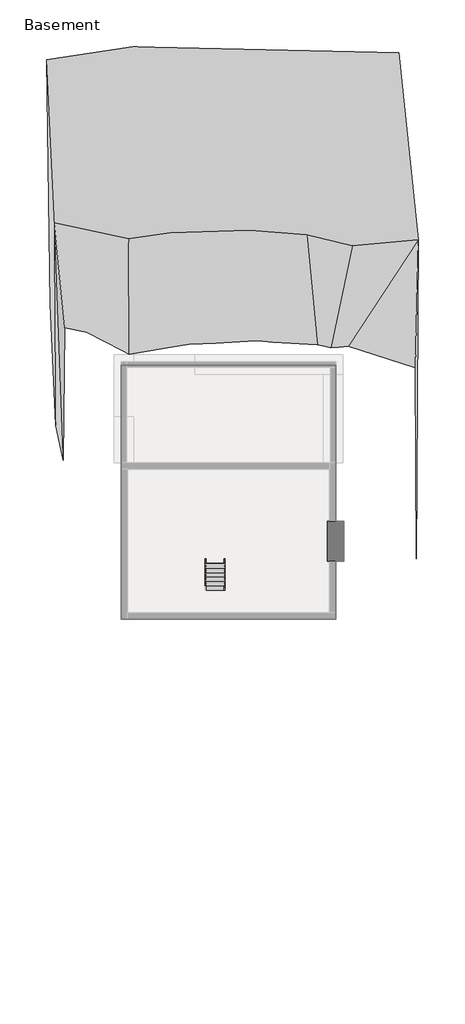
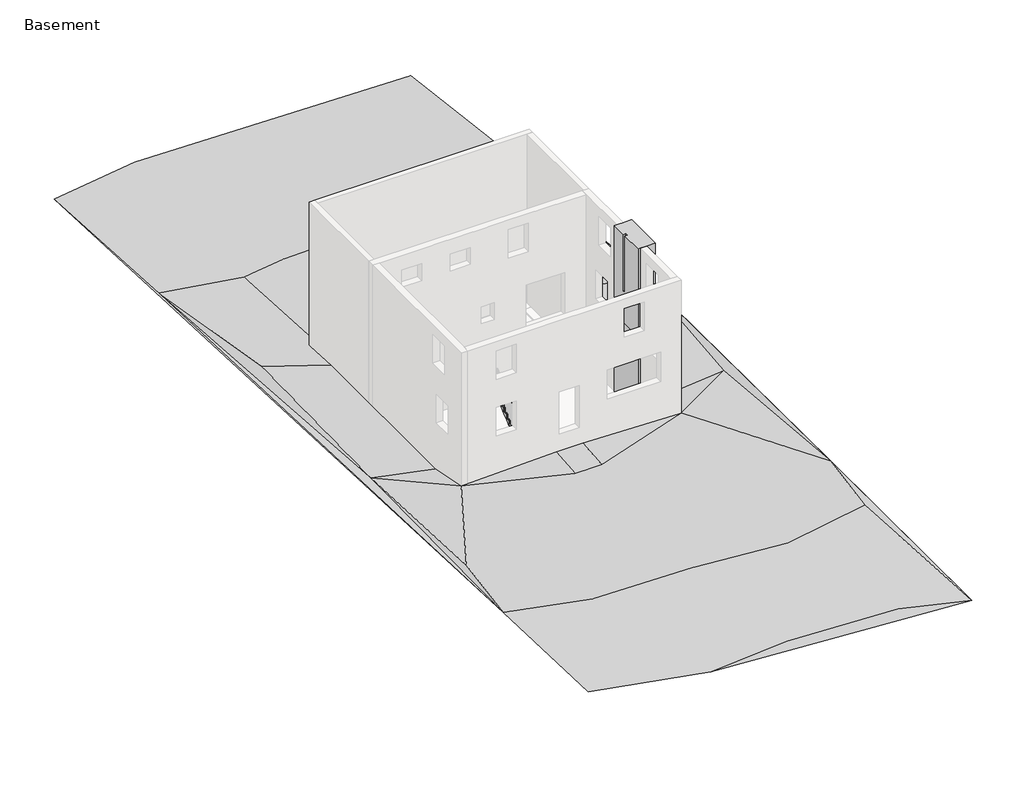
# One storey, part 2 of 2: 4 proxies, 2 members, 1 railing, 1 stair flight.
"""IFC4 building model written with IfcOpenShell, lengths in millimetres."""

import ifcopenshell
import ifcopenshell.guid

model = None  # the IFC model being written
_history = None  # IfcOwnerHistory: only IFC2X3 demands one
_inside = {}  # id of a spatial element -> (the spatial element, [elements in it])
_under = {}  # id of a project, library or spatial element -> (it, [spatial elements below it])
_declared = {}  # id of a project -> (the project, [libraries it declares])
_typed = {}  # id of a type object -> (the type object, [elements of that type])
_made_of = {}  # id of a material, layer set ... -> (it, [elements and type objects made of it])


def new_model(schema):
    """Start an empty IFC model of exactly this schema.

    Asked for "IFC4X3", IfcOpenShell would pick the latest addendum, in which some entities
    have other attributes; the version numbers below select the first issue.
    IFC2X3 requires an IfcOwnerHistory on every rooted entity: one is made here for all.
    """
    global model, _history
    if schema == "IFC4X3":
        model = ifcopenshell.file(schema_version=(4, 3, 0, 0))
    else:
        model = ifcopenshell.file(schema=schema)
    _inside.clear()
    _under.clear()
    _declared.clear()
    _typed.clear()
    _made_of.clear()
    _history = None
    if model.schema == "IFC2X3":
        org = make("IfcOrganization", Name="unknown")
        user = make(
            "IfcPersonAndOrganization",
            ThePerson=make("IfcPerson", FamilyName="unknown"),
            TheOrganization=org,
        )
        app = make(
            "IfcApplication",
            ApplicationDeveloper=org,
            Version="unknown",
            ApplicationFullName="unknown",
            ApplicationIdentifier="unknown",
        )
        _history = make(
            "IfcOwnerHistory",
            OwningUser=user,
            OwningApplication=app,
            ChangeAction="ADDED",
            CreationDate=0,
        )
    return model


def make(cls, **values):
    """One entity of the class cls with the attributes given. An attribute that is None is left unset."""
    return model.create_entity(
        cls, **{name: value for name, value in values.items() if value is not None}
    )


def rooted(cls, **values):
    """An entity with a GlobalId (a new one), such as an element, a storey or a relation."""
    return make(cls, GlobalId=ifcopenshell.guid.new(), OwnerHistory=_history, **values)


def si_unit(unit_type, name, prefix=None):
    """IfcSIUnit, for example si_unit("LENGTHUNIT", "METRE", prefix="MILLI")."""
    return make("IfcSIUnit", UnitType=unit_type, Prefix=prefix, Name=name)


def assignment(units):
    """IfcUnitAssignment: the units of a project."""
    return None if units is None else make("IfcUnitAssignment", Units=units)


def point(xyz):
    """IfcCartesianPoint."""
    return None if xyz is None else make("IfcCartesianPoint", Coordinates=xyz)


def direction(xyz):
    """IfcDirection."""
    return None if xyz is None else make("IfcDirection", DirectionRatios=xyz)


def frame(location, z_axis=None, x_axis=None):
    """IfcAxis2Placement3D, a coordinate frame: its origin and axes. An axis left out is left unset."""
    return make(
        "IfcAxis2Placement3D",
        Location=point(location),
        Axis=direction(z_axis),
        RefDirection=direction(x_axis),
    )


def origin():
    """The frame at (0, 0, 0) with its axes left unset."""
    return frame((0.0, 0.0, 0.0))


def place(relative_to, where):
    """IfcLocalPlacement: puts the frame where relative to a parent placement (None: the world)."""
    return make(
        "IfcLocalPlacement", PlacementRelTo=relative_to, RelativePlacement=where
    )


def context(
    kind, dimensions, precision=None, world=None, true_north=None, identifier=None
):
    """IfcGeometricRepresentationContext, for example the 3D "Model" context."""
    return make(
        "IfcGeometricRepresentationContext",
        ContextIdentifier=identifier,
        ContextType=kind,
        CoordinateSpaceDimension=dimensions,
        Precision=precision,
        WorldCoordinateSystem=world,
        TrueNorth=true_north,
    )


def project(units=None, contexts=None):
    """IfcProject with its units and contexts."""
    return rooted(
        "IfcProject",
        Name="project",
        RepresentationContexts=contexts,
        UnitsInContext=assignment(units),
    )


def spatial(cls, under=None, at=None, **own):
    """A site, building, storey or space (cls), placed at a placement, below another one or the project."""
    s = rooted(cls, ObjectPlacement=at, **own)
    if under is not None:
        _under.setdefault(under.id(), (under, []))[1].append(s)
    return s


def polyline(points):
    """IfcPolyline through the points."""
    return make("IfcPolyline", Points=[point(p) for p in points])


def point_list(points):
    """IfcCartesianPointList2D or 3D."""
    cls = (
        "IfcCartesianPointList2D" if len(points[0]) == 2 else "IfcCartesianPointList3D"
    )
    return make(cls, CoordList=points)


def outline(outer, holes=None, kind="AREA"):
    """IfcArbitraryClosedProfileDef: a profile drawn as a closed curve; with holes, ...WithVoids."""
    if holes is None:
        return make("IfcArbitraryClosedProfileDef", ProfileType=kind, OuterCurve=outer)
    return make(
        "IfcArbitraryProfileDefWithVoids",
        ProfileType=kind,
        OuterCurve=outer,
        InnerCurves=holes,
    )


def extrude(swept, where, along, depth):
    """IfcExtrudedAreaSolid: the profile swept, set in the frame where, extruded along a direction by depth."""
    return make(
        "IfcExtrudedAreaSolid",
        SweptArea=swept,
        Position=where,
        ExtrudedDirection=direction(along),
        Depth=depth,
    )


def faces_of(points, faces, orient=None, outer=None):
    """IfcFace entities. A face is a list of loops; a loop is a list of indices into points, from 0.

    orient and outer hold one flag for each loop. By default every Orientation is true, the
    first loop of a face is its IfcFaceOuterBound and the others are IfcFaceBound.
    """
    made = []
    for i, loops in enumerate(faces):
        bounds = []
        for j, loop in enumerate(loops):
            is_outer = j == 0 if outer is None else outer[i][j]
            bounds.append(
                make(
                    "IfcFaceOuterBound" if is_outer else "IfcFaceBound",
                    Bound=make("IfcPolyLoop", Polygon=[points[k] for k in loop]),
                    Orientation=True if orient is None else orient[i][j],
                )
            )
        made.append(make("IfcFace", Bounds=bounds))
    return made


def faceted_brep(points, faces, orient=None, outer=None, voids=None):
    """IfcFacetedBrep: a solid bounded by flat faces; with voids (closed shells), ...WithVoids."""
    shared = [point(p) for p in points]
    hull = make("IfcClosedShell", CfsFaces=faces_of(shared, faces, orient, outer))
    if voids is None:
        return make("IfcFacetedBrep", Outer=hull)
    return make(
        "IfcFacetedBrepWithVoids",
        Outer=hull,
        Voids=[
            make(cls, CfsFaces=faces_of(shared, fs, o, b)) for cls, fs, o, b in voids
        ],
    )


def triangles(points, corners, closed=None, point_numbers=None):
    """IfcTriangulatedFaceSet: each triangle names its three corners, points numbered from 1."""
    return make(
        "IfcTriangulatedFaceSet",
        Coordinates=point_list(points),
        Closed=closed,
        CoordIndex=corners,
        PnIndex=point_numbers,
    )


def shape(context_of_items, identifier, shape_type, items):
    """IfcShapeRepresentation: the items that make up one representation, for example the "Body"."""
    return make(
        "IfcShapeRepresentation",
        ContextOfItems=context_of_items,
        RepresentationIdentifier=identifier,
        RepresentationType=shape_type,
        Items=items,
    )


def source(mapping_origin, context_of_items, identifier, shape_type, items):
    """IfcRepresentationMap: a shape defined once, which mapped items show again and again."""
    return make(
        "IfcRepresentationMap",
        MappingOrigin=mapping_origin,
        MappedRepresentation=shape(context_of_items, identifier, shape_type, items),
    )


def transform(
    local_origin,
    x_axis=None,
    y_axis=None,
    z_axis=None,
    scale=None,
    scale2=None,
    scale3=None,
    uniform=True,
):
    """IfcCartesianTransformationOperator3D, or its non-uniform kind. x_axis, y_axis, z_axis: its Axis1, 2, 3."""
    if uniform:
        return make(
            "IfcCartesianTransformationOperator3D",
            Axis1=direction(x_axis),
            Axis2=direction(y_axis),
            LocalOrigin=point(local_origin),
            Scale=scale,
            Axis3=direction(z_axis),
        )
    return make(
        "IfcCartesianTransformationOperator3DnonUniform",
        Axis1=direction(x_axis),
        Axis2=direction(y_axis),
        LocalOrigin=point(local_origin),
        Scale=scale,
        Axis3=direction(z_axis),
        Scale2=scale2,
        Scale3=scale3,
    )


def mapped(mapping_source, mapping_target):
    """IfcMappedItem: shows the shape of a source again, moved by a transform."""
    return make(
        "IfcMappedItem", MappingSource=mapping_source, MappingTarget=mapping_target
    )


def made_of(thing, what):
    """Note that an element or type object is made of a material, layer set ...; save() writes the relation."""
    if what is not None:
        _made_of.setdefault(what.id(), (what, []))[1].append(thing)
    return thing


def element(
    cls,
    number,
    at=None,
    inside=None,
    cuts=None,
    type_object=None,
    material=None,
    context=None,
    identifier="Body",
    shape_type=None,
    held_by="IfcProductDefinitionShape",
    body=None,
    shapes=None,
    **own,
):
    """One element of the class cls, such as IfcWall. Its Tag is "e" and its number.

    at: its placement. inside: the storey or other place that contains it. cuts: it is an
    opening in that element (IfcRelVoidsElement). A single representation is given by context,
    identifier, shape_type and body (its items); several are given by shapes. held_by: the class
    of the entity that holds the representations. save() writes the other relations.
    """
    e = rooted(cls, Tag="e%d" % number, ObjectPlacement=at, **own)
    if body is not None:
        shapes = [shape(context, identifier, shape_type, body)]
    if shapes is not None:
        e.Representation = make(held_by, Representations=shapes)
    if inside is not None:
        _inside.setdefault(inside.id(), (inside, []))[1].append(e)
    if cuts is not None:
        rooted(
            "IfcRelVoidsElement", RelatingBuildingElement=cuts, RelatedOpeningElement=e
        )
    if type_object is not None:
        _typed.setdefault(type_object.id(), (type_object, []))[1].append(e)
    return made_of(e, material)


def aggregate(whole, parts):
    """IfcRelAggregates: a whole, such as a stair, and the parts it consists of."""
    return rooted("IfcRelAggregates", RelatingObject=whole, RelatedObjects=parts)


def save(model, path):
    """Write the relations noted so far, then the file.

    IfcRelAggregates (storeys below a building ...), IfcRelContainedInSpatialStructure (elements
    in a storey), IfcRelDefinesByType, IfcRelAssociatesMaterial and IfcRelDeclares: one each for
    every whole, place, type object, material and project.
    """
    for whole, parts in _under.values():
        aggregate(whole, parts)
    for where, things in _inside.values():
        rooted(
            "IfcRelContainedInSpatialStructure",
            RelatedElements=things,
            RelatingStructure=where,
        )
    for kind, things in _typed.values():
        rooted("IfcRelDefinesByType", RelatedObjects=things, RelatingType=kind)
    for what, things in _made_of.values():
        rooted("IfcRelAssociatesMaterial", RelatedObjects=things, RelatingMaterial=what)
    for by, libraries in _declared.values():
        rooted("IfcRelDeclares", RelatingContext=by, RelatedDefinitions=libraries)
    model.write(path)


def existing_fireplace_existing_fireplace_063a625f(model_context):
    return source(origin(), model_context, "Body", "Brep", [
        faceted_brep([(4450.2196932, 434.2888758, 5486.4), (4069.2196932, 434.2888758, 5486.4), (3764.4196932, 434.2888758, 5486.4), (3662.8196932, 434.2888758, 5486.4), (3662.8196932, -276.9111242, 5486.4), (3767.2567114, -276.9111242, 5486.4), (3767.2567114, -403.9111242, 5486.4), (3662.8196932, -403.9111242, 5486.4), (3662.8196932, -1445.3111242, 5486.4), (3764.4196932, -1445.3111242, 5486.4), (4069.2196932, -1445.3111242, 5486.4), (4450.2196932, -1445.3111242, 5486.4), (4450.2196932, 434.2888758, -2667.0), (4450.2196932, -1445.3111242, -2667.0), (4069.2196932, -1445.3111242, -2667.0), (3764.4196932, -1445.3111242, -2667.0), (3662.8196932, -1445.3111242, -2667.0), (3662.8196932, 434.2888758, -2667.0), (3764.4196932, 434.2888758, -2667.0), (4069.2196932, 434.2888758, -2667.0), (3662.8196932, -403.9111242, 2743.2), (3662.8196932, -276.9111242, 2743.2), (3662.8196932, 154.8888758, 0.0), (3662.8196932, 154.8888758, 1219.2), (3662.8196932, -1165.9111242, 1219.2), (3662.8196932, -1165.9111242, 0.0), (4145.4196932, -20.7631592, 1219.2), (4145.4196932, -990.2590891, 1219.2), (4145.4196932, -990.2590891, 0.0), (4145.4196932, -20.7631592, 0.0), (3767.2567114, -403.9111242, 2743.2), (3767.2567114, -276.9111242, 2743.2)], [[[0, 1, 2, 3, 4, 5, 6, 7, 8, 9, 10, 11]], [[12, 13, 14, 15, 16, 17, 18, 19]], [[3, 2, 1, 0, 12, 19, 18, 17]], [[3, 17, 16, 8, 7, 20, 21, 4], [22, 23, 24, 25]], [[11, 10, 9, 8, 16, 15, 14, 13]], [[0, 11, 13, 12]], [[24, 23, 26, 27]], [[25, 24, 27, 28]], [[27, 26, 29, 28]], [[23, 22, 29, 26]], [[22, 25, 28, 29]], [[6, 30, 20, 7]], [[31, 5, 4, 21]], [[30, 31, 21, 20]], [[30, 6, 5, 31]]]),
    ])


def stair_flight_b746b64e(model_context):
    return source(origin(), model_context, "Body", "SweptSolid", [
        extrude(outline(polyline([(-2791.5111242, -2476.5), (-2562.9111242, -2476.5), (-2562.9111242, -2527.3), (-2766.1111242, -2527.3), (-2766.1111242, -2520.95), (-2791.5111242, -2495.55), (-2791.5111242, -2476.5)])), frame((-2052.1803068, 0.0, 0.0), z_axis=(1.0, 0.0, 0.0), x_axis=(0.0, 1.0, 0.0)), (0.0, 0.0, 1.0), 939.8),
        extrude(outline(polyline([(-1112.3803068, -2759.7611242), (-1112.3803068, -2766.1111242), (-2052.1803068, -2766.1111242), (-2052.1803068, -2759.7611242), (-1112.3803068, -2759.7611242)])), frame((0.0, 0.0, -2667.0), z_axis=(0.0, 0.0, 1.0), x_axis=(1.0, 0.0, 0.0)), (0.0, 0.0, 1.0), 139.7),
        extrude(outline(polyline([(-1112.3803068, -2556.5611242), (-1112.3803068, -2562.9111242), (-2052.1803068, -2562.9111242), (-2052.1803068, -2556.5611242), (-1112.3803068, -2556.5611242)])), frame((0.0, 0.0, -2527.3), z_axis=(0.0, 0.0, 1.0), x_axis=(1.0, 0.0, 0.0)), (0.0, 0.0, 1.0), 190.5),
        extrude(outline(polyline([(-2588.3111242, -2286.0), (-2359.7111242, -2286.0), (-2359.7111242, -2336.8), (-2562.9111242, -2336.8), (-2562.9111242, -2330.45), (-2588.3111242, -2305.05), (-2588.3111242, -2286.0)])), frame((-2052.1803068, 0.0, 0.0), z_axis=(1.0, 0.0, 0.0), x_axis=(0.0, 1.0, 0.0)), (0.0, 0.0, 1.0), 939.8),
        extrude(outline(polyline([(-1112.3803068, -2353.3611242), (-1112.3803068, -2359.7111242), (-2052.1803068, -2359.7111242), (-2052.1803068, -2353.3611242), (-1112.3803068, -2353.3611242)])), frame((0.0, 0.0, -2336.8), z_axis=(0.0, 0.0, 1.0), x_axis=(1.0, 0.0, 0.0)), (0.0, 0.0, 1.0), 190.5),
        extrude(outline(polyline([(-2385.1111242, -2095.5), (-2156.5111242, -2095.5), (-2156.5111242, -2146.3), (-2359.7111242, -2146.3), (-2359.7111242, -2139.95), (-2385.1111242, -2114.55), (-2385.1111242, -2095.5)])), frame((-2052.1803068, 0.0, 0.0), z_axis=(1.0, 0.0, 0.0), x_axis=(0.0, 1.0, 0.0)), (0.0, 0.0, 1.0), 939.8),
        extrude(outline(polyline([(-1112.3803068, -2150.1611242), (-1112.3803068, -2156.5111242), (-2052.1803068, -2156.5111242), (-2052.1803068, -2150.1611242), (-1112.3803068, -2150.1611242)])), frame((0.0, 0.0, -2146.3), z_axis=(0.0, 0.0, 1.0), x_axis=(1.0, 0.0, 0.0)), (0.0, 0.0, 1.0), 190.5),
        extrude(outline(polyline([(-2181.9111242, -1905.0), (-1953.3111242, -1905.0), (-1953.3111242, -1955.8), (-2156.5111242, -1955.8), (-2156.5111242, -1949.45), (-2181.9111242, -1924.05), (-2181.9111242, -1905.0)])), frame((-2052.1803068, 0.0, 0.0), z_axis=(1.0, 0.0, 0.0), x_axis=(0.0, 1.0, 0.0)), (0.0, 0.0, 1.0), 939.8),
        extrude(outline(polyline([(-1112.3803068, -1946.9611242), (-1112.3803068, -1953.3111242), (-2052.1803068, -1953.3111242), (-2052.1803068, -1946.9611242), (-1112.3803068, -1946.9611242)])), frame((0.0, 0.0, -1955.8), z_axis=(0.0, 0.0, 1.0), x_axis=(1.0, 0.0, 0.0)), (0.0, 0.0, 1.0), 190.5),
        extrude(outline(polyline([(-1978.7111242, -1714.5), (-1750.1111242, -1714.5), (-1750.1111242, -1765.3), (-1953.3111242, -1765.3), (-1953.3111242, -1758.95), (-1978.7111242, -1733.55), (-1978.7111242, -1714.5)])), frame((-2052.1803068, 0.0, 0.0), z_axis=(1.0, 0.0, 0.0), x_axis=(0.0, 1.0, 0.0)), (0.0, 0.0, 1.0), 939.8),
        extrude(outline(polyline([(-1112.3803068, -1743.7611242), (-1112.3803068, -1750.1111242), (-2052.1803068, -1750.1111242), (-2052.1803068, -1743.7611242), (-1112.3803068, -1743.7611242)])), frame((0.0, 0.0, -1765.3), z_axis=(0.0, 0.0, 1.0), x_axis=(1.0, 0.0, 0.0)), (0.0, 0.0, 1.0), 190.5),
        extrude(outline(polyline([(-1775.5111242, -1524.0), (-1546.9111242, -1524.0), (-1546.9111242, -1574.8), (-1750.1111242, -1574.8), (-1750.1111242, -1568.45), (-1775.5111242, -1543.05), (-1775.5111242, -1524.0)])), frame((-2052.1803068, 0.0, 0.0), z_axis=(1.0, 0.0, 0.0), x_axis=(0.0, 1.0, 0.0)), (0.0, 0.0, 1.0), 939.8),
        extrude(outline(polyline([(-1112.3803068, -1540.5611242), (-1112.3803068, -1546.9111242), (-2052.1803068, -1546.9111242), (-2052.1803068, -1540.5611242), (-1112.3803068, -1540.5611242)])), frame((0.0, 0.0, -1574.8), z_axis=(0.0, 0.0, 1.0), x_axis=(1.0, 0.0, 0.0)), (0.0, 0.0, 1.0), 190.5),
        extrude(outline(polyline([(-1572.3111242, -1333.5), (-1343.7111242, -1333.5), (-1343.7111242, -1384.3), (-1546.9111242, -1384.3), (-1546.9111242, -1377.95), (-1572.3111242, -1352.55), (-1572.3111242, -1333.5)])), frame((-2052.1803068, 0.0, 0.0), z_axis=(1.0, 0.0, 0.0), x_axis=(0.0, 1.0, 0.0)), (0.0, 0.0, 1.0), 939.8),
        extrude(outline(polyline([(-1112.3803068, -1337.3611242), (-1112.3803068, -1343.7111242), (-2052.1803068, -1343.7111242), (-2052.1803068, -1337.3611242), (-1112.3803068, -1337.3611242)])), frame((0.0, 0.0, -1384.3), z_axis=(0.0, 0.0, 1.0), x_axis=(1.0, 0.0, 0.0)), (0.0, 0.0, 1.0), 190.5),
        extrude(outline(polyline([(-1369.1111242, -1143.0), (-1140.5111242, -1143.0), (-1140.5111242, -1193.8), (-1343.7111242, -1193.8), (-1343.7111242, -1187.45), (-1369.1111242, -1162.05), (-1369.1111242, -1143.0)])), frame((-2052.1803068, 0.0, 0.0), z_axis=(1.0, 0.0, 0.0), x_axis=(0.0, 1.0, 0.0)), (0.0, 0.0, 1.0), 939.8),
        extrude(outline(polyline([(-1112.3803068, -1134.1611242), (-1112.3803068, -1140.5111242), (-2052.1803068, -1140.5111242), (-2052.1803068, -1134.1611242), (-1112.3803068, -1134.1611242)])), frame((0.0, 0.0, -1193.8), z_axis=(0.0, 0.0, 1.0), x_axis=(1.0, 0.0, 0.0)), (0.0, 0.0, 1.0), 190.5),
        extrude(outline(polyline([(-1165.9111242, -952.5), (-937.3111242, -952.5), (-937.3111242, -1003.3), (-1140.5111242, -1003.3), (-1140.5111242, -996.95), (-1165.9111242, -971.55), (-1165.9111242, -952.5)])), frame((-2052.1803068, 0.0, 0.0), z_axis=(1.0, 0.0, 0.0), x_axis=(0.0, 1.0, 0.0)), (0.0, 0.0, 1.0), 939.8),
        extrude(outline(polyline([(-1112.3803068, -930.9611242), (-1112.3803068, -937.3111242), (-2052.1803068, -937.3111242), (-2052.1803068, -930.9611242), (-1112.3803068, -930.9611242)])), frame((0.0, 0.0, -1003.3), z_axis=(0.0, 0.0, 1.0), x_axis=(1.0, 0.0, 0.0)), (0.0, 0.0, 1.0), 190.5),
        extrude(outline(polyline([(-962.7111242, -762.0), (-734.1111242, -762.0), (-734.1111242, -812.8), (-937.3111242, -812.8), (-937.3111242, -806.45), (-962.7111242, -781.05), (-962.7111242, -762.0)])), frame((-2052.1803068, 0.0, 0.0), z_axis=(1.0, 0.0, 0.0), x_axis=(0.0, 1.0, 0.0)), (0.0, 0.0, 1.0), 939.8),
        extrude(outline(polyline([(-1112.3803068, -727.7611242), (-1112.3803068, -734.1111242), (-2052.1803068, -734.1111242), (-2052.1803068, -727.7611242), (-1112.3803068, -727.7611242)])), frame((0.0, 0.0, -812.8), z_axis=(0.0, 0.0, 1.0), x_axis=(1.0, 0.0, 0.0)), (0.0, 0.0, 1.0), 190.5),
        extrude(outline(polyline([(-759.5111242, -571.5), (-530.9111242, -571.5), (-530.9111242, -622.3), (-734.1111242, -622.3), (-734.1111242, -615.95), (-759.5111242, -590.55), (-759.5111242, -571.5)])), frame((-2052.1803068, 0.0, 0.0), z_axis=(1.0, 0.0, 0.0), x_axis=(0.0, 1.0, 0.0)), (0.0, 0.0, 1.0), 939.8),
        extrude(outline(polyline([(-1112.3803068, -524.5611242), (-1112.3803068, -530.9111242), (-2052.1803068, -530.9111242), (-2052.1803068, -524.5611242), (-1112.3803068, -524.5611242)])), frame((0.0, 0.0, -622.3), z_axis=(0.0, 0.0, 1.0), x_axis=(1.0, 0.0, 0.0)), (0.0, 0.0, 1.0), 190.5),
        extrude(outline(polyline([(-556.3111242, -381.0), (-327.7111242, -381.0), (-327.7111242, -431.8), (-530.9111242, -431.8), (-530.9111242, -425.45), (-556.3111242, -400.05), (-556.3111242, -381.0)])), frame((-2052.1803068, 0.0, 0.0), z_axis=(1.0, 0.0, 0.0), x_axis=(0.0, 1.0, 0.0)), (0.0, 0.0, 1.0), 939.8),
        extrude(outline(polyline([(-1112.3803068, -321.3611242), (-1112.3803068, -327.7111242), (-2052.1803068, -327.7111242), (-2052.1803068, -321.3611242), (-1112.3803068, -321.3611242)])), frame((0.0, 0.0, -431.8), z_axis=(0.0, 0.0, 1.0), x_axis=(1.0, 0.0, 0.0)), (0.0, 0.0, 1.0), 190.5),
        extrude(outline(polyline([(-353.1111242, -190.5), (-124.5111242, -190.5), (-124.5111242, -241.3), (-327.7111242, -241.3), (-327.7111242, -234.95), (-353.1111242, -209.55), (-353.1111242, -190.5)])), frame((-2052.1803068, 0.0, 0.0), z_axis=(1.0, 0.0, 0.0), x_axis=(0.0, 1.0, 0.0)), (0.0, 0.0, 1.0), 939.8),
        extrude(outline(polyline([(-1112.3803068, -118.1611242), (-1112.3803068, -124.5111242), (-2052.1803068, -124.5111242), (-2052.1803068, -118.1611242), (-1112.3803068, -118.1611242)])), frame((0.0, 0.0, -241.3), z_axis=(0.0, 0.0, 1.0), x_axis=(1.0, 0.0, 0.0)), (0.0, 0.0, 1.0), 190.5),
    ])


model = new_model("IFC4")

# Units and contexts
model_context = context("Model", 3, world=origin())
ifc_project = project(units=[si_unit("LENGTHUNIT", "METRE", prefix="MILLI")], contexts=[model_context])

# Site, building, storey
site = spatial("IfcSite", under=ifc_project)
building = spatial("IfcBuilding", under=site)
storey = spatial("IfcBuildingStorey", under=building, Name="Basement", Elevation=-2667.0)

# Proxies
placement = place(None, origin())
element("IfcBuildingElementProxy", 1, Name="Building Element Proxy", at=placement, inside=storey, context=model_context, shape_type="Tessellation", body=[
    triangles([(-9474.14729, 22003.2871765, -1727.1999516), (-8916.1412338, -12566.1132111, -939.7999758), (-8632.7724838, -18803.3999359, -1092.1999758), (-3754.3850807, -20036.8885986, -1092.1999758), (7677.2023224, -20906.8378235, -1092.1999758), (7936.7585724, 13587.9496765, -1752.6), (7012.0400162, 22339.8364014, -1727.1999516), (-5437.1349838, 22620.8239014, -1727.1999516), (4069.2196426, 434.2888621, -1346.1999516), (4450.2196426, 434.2888621, -1346.1999516), (4450.2196426, -349.5066825, -1346.1999516), (4450.2196426, -1445.3110531, -1346.1999516), (4069.2196426, -1445.3110531, -1346.1999516), (4069.2196426, -2313.9084709, -1346.1999516), (4069.2196426, -4163.1110046, -939.7999758), (-426.580321, -4163.1110046, -812.8000242), (-1645.7803574, -4163.1110046, -812.8000242), (-5989.1803574, -4163.1110046, -939.7999758), (-5989.1803574, -2124.4043404, -1346.1999516), (-5989.1803574, 3152.0889954, -1346.1999516), (-5989.1803574, 4989.0600082, -1346.1999516), (-5989.1803574, 6156.3282944, -1346.1999516), (-5989.1803574, 7724.0889954, -1429.2445919), (-5611.7969971, 7724.0889954, -1439.6358181), (-2815.8938187, 7724.0889954, -1415.0254017), (-2474.4123367, 7724.0889954, -1412.4145145), (-1876.9665367, 7724.0889954, -1411.4359406), (391.3462071, 7724.0889954, -1403.6252254), (781.867392, 7724.0889954, -1405.4288944), (3306.7437996, 7724.0889954, -1413.4377079), (3676.8014442, 7724.0889954, -1418.4369667), (4069.2196426, 7724.0889954, -1416.2554138), (4069.2196426, 7529.9159637, -1404.4058464), (4069.2196426, 6299.0253983, -1346.1999516), (4069.2196426, 3152.0889954, -1346.1999516), (-9109.81604, 14372.1750641, -1752.6), (-8549.4287338, -9013.2876297, -939.7999758), (-8523.2349838, -1401.2252266, -1346.1999516), (-8408.9349838, 7414.1625641, -1346.1999516), (-6082.4537338, -10022.9382111, -939.7999758), (-5633.19104, 13643.5125641, -1752.6), (-5382.3662338, -13518.6132111, -939.7999758), (-3671.0413307, 13924.5000641, -1752.6), (-2942.3788307, -9965.7882111, -939.7999758), (-1568.3975807, 21947.7254517, -1727.1999516), (-840.5287823, -13629.7378235, -939.7999758), (-699.241258, -10470.6132111, -939.7999758), (-109.4850414, -19700.3370483, -1092.1999758), (29.4212079, 14035.6246765, -1752.6), (2721.8210724, 13811.7871765, -1752.6), (2805.1648224, 21892.1614014, -1727.1999516), (3252.0462662, -14021.8499359, -939.7999758), (4179.1460724, -9854.6624359, -939.7999758), (4845.1025162, -19962.2745483, -1092.1999758), (4852.2462662, 13306.9621765, -1752.6), (7177.93396, -13294.7757111, -939.7999758), (7289.85271, -1961.6126781, -1346.1999516), (7543.0587662, -9965.7882111, -939.7999758), (7740.7025162, 5059.8998703, -1346.1999516), (-1645.7803574, -5668.0610046, -939.7999758), (-426.580321, -5668.0610046, -939.7999758)], [[40, 2, 42], [42, 2, 3], [2, 40, 37], [37, 38, 2], [38, 37, 18], [18, 19, 38], [37, 40, 18], [38, 19, 20], [40, 60, 18], [2, 38, 36], [42, 4, 46], [4, 42, 3], [42, 46, 44], [47, 46, 52], [4, 48, 46], [44, 46, 47], [60, 17, 18], [44, 47, 60], [61, 16, 17], [17, 60, 61], [40, 44, 60], [60, 47, 61], [44, 40, 42], [21, 22, 39], [20, 21, 39], [8, 1, 36], [36, 1, 2], [36, 39, 41], [23, 39, 22], [36, 38, 39], [23, 41, 39], [20, 39, 38], [41, 24, 25], [25, 26, 43], [27, 43, 26], [41, 8, 36], [8, 41, 43], [43, 45, 8], [49, 45, 43], [41, 25, 43], [8, 45, 51], [49, 43, 27], [24, 41, 23], [52, 53, 47], [52, 48, 54], [53, 52, 56], [47, 53, 61], [14, 15, 57], [61, 53, 15], [13, 14, 12], [58, 15, 53], [52, 46, 48], [56, 58, 53], [56, 54, 5], [58, 5, 59], [5, 58, 56], [54, 48, 5], [58, 57, 15], [10, 11, 57], [12, 57, 11], [12, 14, 57], [10, 57, 59], [58, 59, 57], [56, 52, 54], [48, 4, 5], [49, 28, 29], [50, 29, 30], [49, 50, 51], [49, 29, 50], [31, 55, 30], [50, 55, 51], [50, 30, 55], [49, 51, 45], [49, 27, 28], [34, 35, 59], [33, 59, 32], [59, 33, 34], [9, 10, 35], [32, 55, 31], [55, 32, 6], [6, 7, 55], [32, 59, 6], [55, 7, 51], [59, 5, 6], [10, 59, 35], [51, 7, 8], [16, 61, 15]], closed=False),
])
element("IfcBuildingElementProxy", 2, Name="Building Element Proxy", at=placement, inside=storey, context=model_context, shape_type="Tessellation", body=[
    triangles([(4069.2196426, 3152.0889954, -3073.5594864), (4069.2196426, 3152.0889954, -1346.1999516), (4069.2196426, 434.2888621, -3073.5594864), (4069.2196426, 434.2888621, -1346.1999516), (4450.2196426, 434.2888621, -3073.5594864), (4450.2196426, 434.2888621, -1346.1999516), (4450.2196426, -349.5066825, -3073.5594864), (4450.2196426, -349.5066825, -1346.1999516), (4450.2196426, -1445.3110531, -3073.5594864), (4450.2196426, -1445.3110531, -1346.1999516), (4069.2196426, -1445.3110531, -3073.5594864), (4069.2196426, -1445.3110531, -1346.1999516), (4069.2196426, -2313.9084709, -3073.5594864), (4069.2196426, -2313.9084709, -1346.1999516), (4069.2196426, -4163.1110046, -3073.5594864), (4069.2196426, -4163.1110046, -939.7999758), (-426.580321, -4163.1110046, -3073.5594864), (-426.580321, -4163.1110046, -812.8000242), (-1645.7803574, -4163.1110046, -3073.5594864), (-1645.7803574, -4163.1110046, -812.8000242), (-5989.1803574, -4163.1110046, -3073.5594864), (-5989.1803574, -4163.1110046, -939.7999758), (-5989.1803574, -2124.4043404, -3073.5594864), (-5989.1803574, -2124.4043404, -1346.1999516), (-5989.1803574, 3152.0889954, -3073.5594864), (-5989.1803574, 3152.0889954, -1346.1999516)], [[1, 4, 2], [1, 3, 4], [3, 6, 4], [3, 5, 6], [5, 8, 6], [5, 7, 8], [7, 10, 8], [7, 9, 10], [9, 12, 10], [9, 11, 12], [11, 14, 12], [11, 13, 14], [13, 16, 14], [13, 15, 16], [15, 18, 16], [15, 17, 18], [17, 20, 18], [17, 19, 20], [19, 22, 20], [19, 21, 22], [21, 24, 22], [21, 23, 24], [23, 26, 24], [23, 25, 26]], closed=False),
    triangles([(4069.2196426, 434.2888621, -3073.5594864), (4069.2196426, 3152.0889954, -3073.5594864), (-5989.1803574, 3152.0889954, -3073.5594864), (-5989.1803574, -4163.1110046, -3073.5594864), (4069.2196426, -4163.1110046, -3073.5594864), (4069.2196426, -1445.3110531, -3073.5594864), (4450.2196426, -1445.3110531, -3073.5594864), (4450.2196426, 434.2888621, -3073.5594864)], [[4, 6, 3], [6, 4, 5], [3, 1, 2], [1, 3, 6], [6, 7, 1], [8, 1, 7]], closed=False),
])
element("IfcBuildingElementProxy", 3, Name="Building Element Proxy", at=placement, inside=storey, context=model_context, shape_type="Tessellation", body=[
    triangles([(-5989.1803574, 3152.0889954, -3073.5594864), (-5989.1803574, 3152.0889954, -1346.1999516), (-5989.1803574, 4989.0600082, -3073.5594864), (-5989.1803574, 4989.0600082, -1346.1999516), (-5989.1803574, 6156.3282944, -3073.5594864), (-5989.1803574, 6156.3282944, -1346.1999516), (-5989.1803574, 7724.0889954, -3073.5594864), (-5989.1803574, 7724.0889954, -1429.2445919), (-5611.7969971, 7724.0889954, -3073.5594864), (-5611.7969971, 7724.0889954, -1439.6358181), (-2815.8938187, 7724.0889954, -3073.5594864), (-2815.8938187, 7724.0889954, -1415.0254017), (-2474.4123367, 7724.0889954, -3073.5594864), (-2474.4123367, 7724.0889954, -1412.4145145), (-1876.9665367, 7724.0889954, -3073.5594864), (-1876.9665367, 7724.0889954, -1411.4359406), (391.3462071, 7724.0889954, -3073.5594864), (391.3462071, 7724.0889954, -1403.6252254), (781.867392, 7724.0889954, -3073.5594864), (781.867392, 7724.0889954, -1405.4288944), (3306.7437996, 7724.0889954, -3073.5594864), (3306.7437996, 7724.0889954, -1413.4377079), (3676.8014442, 7724.0889954, -3073.5594864), (3676.8014442, 7724.0889954, -1418.4369667), (4069.2196426, 7724.0889954, -3073.5594864), (4069.2196426, 7724.0889954, -1416.2554138), (4069.2196426, 7529.9159637, -3073.5594864), (4069.2196426, 7529.9159637, -1404.4058464), (4069.2196426, 6299.0253983, -3073.5594864), (4069.2196426, 6299.0253983, -1346.1999516), (4069.2196426, 3152.0889954, -3073.5594864), (4069.2196426, 3152.0889954, -1346.1999516)], [[1, 4, 2], [1, 3, 4], [3, 6, 4], [3, 5, 6], [5, 8, 6], [5, 7, 8], [7, 10, 8], [7, 9, 10], [9, 12, 10], [9, 11, 12], [11, 14, 12], [11, 13, 14], [13, 16, 14], [13, 15, 16], [15, 18, 16], [15, 17, 18], [17, 20, 18], [17, 19, 20], [19, 22, 20], [19, 21, 22], [21, 24, 22], [21, 23, 24], [23, 26, 24], [23, 25, 26], [25, 28, 26], [25, 27, 28], [27, 30, 28], [27, 29, 30], [29, 32, 30], [29, 31, 32]], closed=False),
    triangles([(-5989.1803574, 7724.0889954, -3073.5594864), (-5989.1803574, 3152.0889954, -3073.5594864), (4069.2196426, 3152.0889954, -3073.5594864), (4069.2196426, 7724.0889954, -3073.5594864)], [[1, 2, 4], [3, 4, 2]], closed=False),
])
existing_fireplace_existing_fireplace_shape = existing_fireplace_existing_fireplace_063a625f(model_context)
element("IfcBuildingElementProxy", 4, Name="Existing Fireplace : Existing Fireplace", ObjectType="Existing Fireplace : Existing Fireplace", at=placement, inside=storey, context=model_context, shape_type="MappedRepresentation", body=[
    mapped(existing_fireplace_existing_fireplace_shape, transform((0.0, 0.0, 0.0), x_axis=(1.0, 0.0, 0.0), y_axis=(0.0, 1.0, 0.0), z_axis=(0.0, 0.0, 1.0))),
])

# Members
element("IfcMember", 5, at=placement, inside=storey, context=model_context, shape_type="Brep", body=[
    faceted_brep([(-2052.1803068, -2759.7611242, -2667.0), (-2052.1803068, -2612.7302092, -2667.0), (-2001.3803068, -2612.7302092, -2667.0), (-2001.3803068, -2759.7611242, -2667.0), (-2001.3803068, -149.9111242, -358.1071078), (-2052.1803068, -149.9111242, -358.1071078), (-2052.1803068, -149.9111242, -241.3), (-2001.3803068, -149.9111242, -241.3), (-2052.1803068, -2556.5611242, -2614.3414828), (-2052.1803068, -2353.3611242, -2423.8414828), (-2052.1803068, -2150.1611242, -2233.3414828), (-2052.1803068, -1946.9611242, -2042.8414828), (-2052.1803068, -1743.7611242, -1852.3414828), (-2052.1803068, -1540.5611242, -1661.8414828), (-2052.1803068, -1337.3611242, -1471.3414828), (-2052.1803068, -1134.1611242, -1280.8414828), (-2052.1803068, -930.9611242, -1090.3414828), (-2052.1803068, -727.7611242, -899.8414828), (-2052.1803068, -524.5611242, -709.3414828), (-2052.1803068, -321.3611242, -518.8414828), (-2052.1803068, -2759.7611242, -2527.3), (-2052.1803068, -2556.5611242, -2527.3), (-2052.1803068, -2556.5611242, -2336.8), (-2052.1803068, -2353.3611242, -2336.8), (-2052.1803068, -2353.3611242, -2146.3), (-2052.1803068, -2150.1611242, -2146.3), (-2052.1803068, -2150.1611242, -1955.8), (-2052.1803068, -1946.9611242, -1955.8), (-2052.1803068, -1946.9611242, -1765.3), (-2052.1803068, -1743.7611242, -1765.3), (-2052.1803068, -1743.7611242, -1574.8), (-2052.1803068, -1540.5611242, -1574.8), (-2052.1803068, -1540.5611242, -1384.3), (-2052.1803068, -1337.3611242, -1384.3), (-2052.1803068, -1337.3611242, -1193.8), (-2052.1803068, -1134.1611242, -1193.8), (-2052.1803068, -1134.1611242, -1003.3), (-2052.1803068, -930.9611242, -1003.3), (-2052.1803068, -930.9611242, -812.8), (-2052.1803068, -727.7611242, -812.8), (-2052.1803068, -727.7611242, -622.3), (-2052.1803068, -524.5611242, -622.3), (-2052.1803068, -524.5611242, -431.8), (-2052.1803068, -321.3611242, -431.8), (-2052.1803068, -321.3611242, -241.3), (-2001.3803068, -321.3611242, -241.3), (-2001.3803068, -321.3611242, -431.8), (-2001.3803068, -524.5611242, -431.8), (-2001.3803068, -524.5611242, -622.3), (-2001.3803068, -727.7611242, -622.3), (-2001.3803068, -727.7611242, -812.8), (-2001.3803068, -930.9611242, -812.8), (-2001.3803068, -930.9611242, -1003.3), (-2001.3803068, -1134.1611242, -1003.3), (-2001.3803068, -1134.1611242, -1193.8), (-2001.3803068, -1337.3611242, -1193.8), (-2001.3803068, -1337.3611242, -1384.3), (-2001.3803068, -1540.5611242, -1384.3), (-2001.3803068, -1540.5611242, -1574.8), (-2001.3803068, -1743.7611242, -1574.8), (-2001.3803068, -1743.7611242, -1765.3), (-2001.3803068, -1946.9611242, -1765.3), (-2001.3803068, -1946.9611242, -1955.8), (-2001.3803068, -2150.1611242, -1955.8), (-2001.3803068, -2150.1611242, -2146.3), (-2001.3803068, -2353.3611242, -2146.3), (-2001.3803068, -2353.3611242, -2336.8), (-2001.3803068, -2556.5611242, -2336.8), (-2001.3803068, -2556.5611242, -2527.3), (-2001.3803068, -2759.7611242, -2527.3)], [[[0, 1, 2, 3]], [[4, 5, 6, 7]], [[5, 4, 2, 1, 8, 9, 10, 11, 12, 13, 14, 15, 16, 17, 18, 19]], [[6, 5, 19, 18, 17, 16, 15, 14, 13, 12, 11, 10, 9, 8, 1, 0, 20, 21, 22, 23, 24, 25, 26, 27, 28, 29, 30, 31, 32, 33, 34, 35, 36, 37, 38, 39, 40, 41, 42, 43, 44]], [[44, 45, 7, 6]], [[4, 7, 45, 46, 47, 48, 49, 50, 51, 52, 53, 54, 55, 56, 57, 58, 59, 60, 61, 62, 63, 64, 65, 66, 67, 68, 69, 3, 2]], [[69, 20, 0, 3]], [[20, 69, 68, 21]], [[21, 68, 67, 22]], [[22, 67, 66, 23]], [[23, 66, 65, 24]], [[24, 65, 64, 25]], [[25, 64, 63, 26]], [[26, 63, 62, 27]], [[27, 62, 61, 28]], [[28, 61, 60, 29]], [[29, 60, 59, 30]], [[30, 59, 58, 31]], [[31, 58, 57, 32]], [[32, 57, 56, 33]], [[33, 56, 55, 34]], [[34, 55, 54, 35]], [[35, 54, 53, 36]], [[36, 53, 52, 37]], [[37, 52, 51, 38]], [[38, 51, 50, 39]], [[39, 50, 49, 40]], [[40, 49, 48, 41]], [[41, 48, 47, 42]], [[42, 47, 46, 43]], [[43, 46, 45, 44]]]),
])
element("IfcMember", 6, at=placement, inside=storey, context=model_context, shape_type="Brep", body=[
    faceted_brep([(-1163.1803068, -2759.7611242, -2667.0), (-1163.1803068, -2612.7302092, -2667.0), (-1112.3803068, -2612.7302092, -2667.0), (-1112.3803068, -2759.7611242, -2667.0), (-1112.3803068, -149.9111242, -358.1071078), (-1163.1803068, -149.9111242, -358.1071078), (-1163.1803068, -149.9111242, -241.3), (-1112.3803068, -149.9111242, -241.3), (-1112.3803068, -321.3611242, -518.8414828), (-1112.3803068, -524.5611242, -709.3414828), (-1112.3803068, -727.7611242, -899.8414828), (-1112.3803068, -930.9611242, -1090.3414828), (-1112.3803068, -1134.1611242, -1280.8414828), (-1112.3803068, -1337.3611242, -1471.3414828), (-1112.3803068, -1540.5611242, -1661.8414828), (-1112.3803068, -1743.7611242, -1852.3414828), (-1112.3803068, -1946.9611242, -2042.8414828), (-1112.3803068, -2150.1611242, -2233.3414828), (-1112.3803068, -2353.3611242, -2423.8414828), (-1112.3803068, -2556.5611242, -2614.3414828), (-1163.1803068, -2759.7611242, -2527.3), (-1163.1803068, -2556.5611242, -2527.3), (-1163.1803068, -2556.5611242, -2336.8), (-1163.1803068, -2353.3611242, -2336.8), (-1163.1803068, -2353.3611242, -2146.3), (-1163.1803068, -2150.1611242, -2146.3), (-1163.1803068, -2150.1611242, -1955.8), (-1163.1803068, -1946.9611242, -1955.8), (-1163.1803068, -1946.9611242, -1765.3), (-1163.1803068, -1743.7611242, -1765.3), (-1163.1803068, -1743.7611242, -1574.8), (-1163.1803068, -1540.5611242, -1574.8), (-1163.1803068, -1540.5611242, -1384.3), (-1163.1803068, -1337.3611242, -1384.3), (-1163.1803068, -1337.3611242, -1193.8), (-1163.1803068, -1134.1611242, -1193.8), (-1163.1803068, -1134.1611242, -1003.3), (-1163.1803068, -930.9611242, -1003.3), (-1163.1803068, -930.9611242, -812.8), (-1163.1803068, -727.7611242, -812.8), (-1163.1803068, -727.7611242, -622.3), (-1163.1803068, -524.5611242, -622.3), (-1163.1803068, -524.5611242, -431.8), (-1163.1803068, -321.3611242, -431.8), (-1163.1803068, -321.3611242, -241.3), (-1112.3803068, -321.3611242, -241.3), (-1112.3803068, -321.3611242, -431.8), (-1112.3803068, -524.5611242, -431.8), (-1112.3803068, -524.5611242, -622.3), (-1112.3803068, -727.7611242, -622.3), (-1112.3803068, -727.7611242, -812.8), (-1112.3803068, -930.9611242, -812.8), (-1112.3803068, -930.9611242, -1003.3), (-1112.3803068, -1134.1611242, -1003.3), (-1112.3803068, -1134.1611242, -1193.8), (-1112.3803068, -1337.3611242, -1193.8), (-1112.3803068, -1337.3611242, -1384.3), (-1112.3803068, -1540.5611242, -1384.3), (-1112.3803068, -1540.5611242, -1574.8), (-1112.3803068, -1743.7611242, -1574.8), (-1112.3803068, -1743.7611242, -1765.3), (-1112.3803068, -1946.9611242, -1765.3), (-1112.3803068, -1946.9611242, -1955.8), (-1112.3803068, -2150.1611242, -1955.8), (-1112.3803068, -2150.1611242, -2146.3), (-1112.3803068, -2353.3611242, -2146.3), (-1112.3803068, -2353.3611242, -2336.8), (-1112.3803068, -2556.5611242, -2336.8), (-1112.3803068, -2556.5611242, -2527.3), (-1112.3803068, -2759.7611242, -2527.3)], [[[0, 1, 2, 3]], [[4, 5, 6, 7]], [[5, 4, 8, 9, 10, 11, 12, 13, 14, 15, 16, 17, 18, 19, 2, 1]], [[6, 5, 1, 0, 20, 21, 22, 23, 24, 25, 26, 27, 28, 29, 30, 31, 32, 33, 34, 35, 36, 37, 38, 39, 40, 41, 42, 43, 44]], [[44, 45, 7, 6]], [[4, 7, 45, 46, 47, 48, 49, 50, 51, 52, 53, 54, 55, 56, 57, 58, 59, 60, 61, 62, 63, 64, 65, 66, 67, 68, 69, 3, 2, 19, 18, 17, 16, 15, 14, 13, 12, 11, 10, 9, 8]], [[69, 20, 0, 3]], [[20, 69, 68, 21]], [[21, 68, 67, 22]], [[22, 67, 66, 23]], [[23, 66, 65, 24]], [[24, 65, 64, 25]], [[25, 64, 63, 26]], [[26, 63, 62, 27]], [[27, 62, 61, 28]], [[28, 61, 60, 29]], [[29, 60, 59, 30]], [[30, 59, 58, 31]], [[31, 58, 57, 32]], [[32, 57, 56, 33]], [[33, 56, 55, 34]], [[34, 55, 54, 35]], [[35, 54, 53, 36]], [[36, 53, 52, 37]], [[37, 52, 51, 38]], [[38, 51, 50, 39]], [[39, 50, 49, 40]], [[40, 49, 48, 41]], [[41, 48, 47, 42]], [[42, 47, 46, 43]], [[43, 46, 45, 44]]]),
])

# Railing
element("IfcRailing", 7, ObjectType="Handrail - Rectangular", at=placement, inside=storey, context=model_context, shape_type="SweptSolid", body=[
    extrude(outline(polyline([(-2791.5111242, -1631.7331862), (-2791.5111242, -1562.1), (-149.9111242, 914.4), (-149.9111242, 844.7668138), (-2791.5111242, -1631.7331862)])), frame((-1163.1803068, 0.0, 0.0), z_axis=(1.0, 0.0, 0.0), x_axis=(0.0, 1.0, 0.0)), (0.0, 0.0, 1.0), 50.8),
    extrude(outline(polyline([(-261.0361242, 740.5871263), (-241.9861242, 758.4465013), (-241.9861242, -190.5), (-261.0361242, -190.5), (-261.0361242, 740.5871263)])), frame((-1147.3053068, 0.0, 0.0), z_axis=(1.0, 0.0, 0.0), x_axis=(0.0, 1.0, 0.0)), (0.0, 0.0, 1.0), 19.05),
    extrude(outline(polyline([(-362.6361242, 645.3371263), (-343.5861242, 663.1965013), (-343.5861242, -190.5), (-362.6361242, -190.5), (-362.6361242, 645.3371263)])), frame((-1147.3053068, 0.0, 0.0), z_axis=(1.0, 0.0, 0.0), x_axis=(0.0, 1.0, 0.0)), (0.0, 0.0, 1.0), 19.05),
    extrude(outline(polyline([(-464.2361242, 550.0871263), (-445.1861242, 567.9465013), (-445.1861242, -381.0), (-464.2361242, -381.0), (-464.2361242, 550.0871263)])), frame((-1147.3053068, 0.0, 0.0), z_axis=(1.0, 0.0, 0.0), x_axis=(0.0, 1.0, 0.0)), (0.0, 0.0, 1.0), 19.05),
    extrude(outline(polyline([(-565.8361242, 454.8371263), (-546.7861242, 472.6965013), (-546.7861242, -381.0), (-565.8361242, -381.0), (-565.8361242, 454.8371263)])), frame((-1147.3053068, 0.0, 0.0), z_axis=(1.0, 0.0, 0.0), x_axis=(0.0, 1.0, 0.0)), (0.0, 0.0, 1.0), 19.05),
    extrude(outline(polyline([(-667.4361242, 359.5871263), (-648.3861242, 377.4465013), (-648.3861242, -571.5), (-667.4361242, -571.5), (-667.4361242, 359.5871263)])), frame((-1147.3053068, 0.0, 0.0), z_axis=(1.0, 0.0, 0.0), x_axis=(0.0, 1.0, 0.0)), (0.0, 0.0, 1.0), 19.05),
    extrude(outline(polyline([(-769.0361242, 264.3371263), (-749.9861242, 282.1965013), (-749.9861242, -571.5), (-769.0361242, -571.5), (-769.0361242, 264.3371263)])), frame((-1147.3053068, 0.0, 0.0), z_axis=(1.0, 0.0, 0.0), x_axis=(0.0, 1.0, 0.0)), (0.0, 0.0, 1.0), 19.05),
    extrude(outline(polyline([(-870.6361242, 169.0871263), (-851.5861242, 186.9465013), (-851.5861242, -762.0), (-870.6361242, -762.0), (-870.6361242, 169.0871263)])), frame((-1147.3053068, 0.0, 0.0), z_axis=(1.0, 0.0, 0.0), x_axis=(0.0, 1.0, 0.0)), (0.0, 0.0, 1.0), 19.05),
    extrude(outline(polyline([(-972.2361242, 73.8371263), (-953.1861242, 91.6965013), (-953.1861242, -762.0), (-972.2361242, -762.0), (-972.2361242, 73.8371263)])), frame((-1147.3053068, 0.0, 0.0), z_axis=(1.0, 0.0, 0.0), x_axis=(0.0, 1.0, 0.0)), (0.0, 0.0, 1.0), 19.05),
    extrude(outline(polyline([(-1073.8361242, -21.4128737), (-1054.7861242, -3.5534987), (-1054.7861242, -952.5), (-1073.8361242, -952.5), (-1073.8361242, -21.4128737)])), frame((-1147.3053068, 0.0, 0.0), z_axis=(1.0, 0.0, 0.0), x_axis=(0.0, 1.0, 0.0)), (0.0, 0.0, 1.0), 19.05),
    extrude(outline(polyline([(-1175.4361242, -116.6628737), (-1156.3861242, -98.8034987), (-1156.3861242, -952.5), (-1175.4361242, -952.5), (-1175.4361242, -116.6628737)])), frame((-1147.3053068, 0.0, 0.0), z_axis=(1.0, 0.0, 0.0), x_axis=(0.0, 1.0, 0.0)), (0.0, 0.0, 1.0), 19.05),
    extrude(outline(polyline([(-1277.0361242, -211.9128737), (-1257.9861242, -194.0534987), (-1257.9861242, -1143.0), (-1277.0361242, -1143.0), (-1277.0361242, -211.9128737)])), frame((-1147.3053068, 0.0, 0.0), z_axis=(1.0, 0.0, 0.0), x_axis=(0.0, 1.0, 0.0)), (0.0, 0.0, 1.0), 19.05),
    extrude(outline(polyline([(-1378.6361242, -307.1628737), (-1359.5861242, -289.3034987), (-1359.5861242, -1143.0), (-1378.6361242, -1143.0), (-1378.6361242, -307.1628737)])), frame((-1147.3053068, 0.0, 0.0), z_axis=(1.0, 0.0, 0.0), x_axis=(0.0, 1.0, 0.0)), (0.0, 0.0, 1.0), 19.05),
    extrude(outline(polyline([(-1480.2361242, -402.4128737), (-1461.1861242, -384.5534987), (-1461.1861242, -1333.5), (-1480.2361242, -1333.5), (-1480.2361242, -402.4128737)])), frame((-1147.3053068, 0.0, 0.0), z_axis=(1.0, 0.0, 0.0), x_axis=(0.0, 1.0, 0.0)), (0.0, 0.0, 1.0), 19.05),
    extrude(outline(polyline([(-1581.8361242, -497.6628737), (-1562.7861242, -479.8034987), (-1562.7861242, -1333.5), (-1581.8361242, -1333.5), (-1581.8361242, -497.6628737)])), frame((-1147.3053068, 0.0, 0.0), z_axis=(1.0, 0.0, 0.0), x_axis=(0.0, 1.0, 0.0)), (0.0, 0.0, 1.0), 19.05),
    extrude(outline(polyline([(-1683.4361242, -592.9128737), (-1664.3861242, -575.0534987), (-1664.3861242, -1524.0), (-1683.4361242, -1524.0), (-1683.4361242, -592.9128737)])), frame((-1147.3053068, 0.0, 0.0), z_axis=(1.0, 0.0, 0.0), x_axis=(0.0, 1.0, 0.0)), (0.0, 0.0, 1.0), 19.05),
    extrude(outline(polyline([(-1785.0361242, -688.1628737), (-1765.9861242, -670.3034987), (-1765.9861242, -1524.0), (-1785.0361242, -1524.0), (-1785.0361242, -688.1628737)])), frame((-1147.3053068, 0.0, 0.0), z_axis=(1.0, 0.0, 0.0), x_axis=(0.0, 1.0, 0.0)), (0.0, 0.0, 1.0), 19.05),
    extrude(outline(polyline([(-1886.6361242, -783.4128737), (-1867.5861242, -765.5534987), (-1867.5861242, -1714.5), (-1886.6361242, -1714.5), (-1886.6361242, -783.4128737)])), frame((-1147.3053068, 0.0, 0.0), z_axis=(1.0, 0.0, 0.0), x_axis=(0.0, 1.0, 0.0)), (0.0, 0.0, 1.0), 19.05),
    extrude(outline(polyline([(-1988.2361242, -878.6628737), (-1969.1861242, -860.8034987), (-1969.1861242, -1714.5), (-1988.2361242, -1714.5), (-1988.2361242, -878.6628737)])), frame((-1147.3053068, 0.0, 0.0), z_axis=(1.0, 0.0, 0.0), x_axis=(0.0, 1.0, 0.0)), (0.0, 0.0, 1.0), 19.05),
    extrude(outline(polyline([(-2089.8361242, -973.9128737), (-2070.7861242, -956.0534987), (-2070.7861242, -1905.0), (-2089.8361242, -1905.0), (-2089.8361242, -973.9128737)])), frame((-1147.3053068, 0.0, 0.0), z_axis=(1.0, 0.0, 0.0), x_axis=(0.0, 1.0, 0.0)), (0.0, 0.0, 1.0), 19.05),
    extrude(outline(polyline([(-2191.4361242, -1069.1628737), (-2172.3861242, -1051.3034987), (-2172.3861242, -1905.0), (-2191.4361242, -1905.0), (-2191.4361242, -1069.1628737)])), frame((-1147.3053068, 0.0, 0.0), z_axis=(1.0, 0.0, 0.0), x_axis=(0.0, 1.0, 0.0)), (0.0, 0.0, 1.0), 19.05),
    extrude(outline(polyline([(-2293.0361242, -1164.4128737), (-2273.9861242, -1146.5534987), (-2273.9861242, -2095.5), (-2293.0361242, -2095.5), (-2293.0361242, -1164.4128737)])), frame((-1147.3053068, 0.0, 0.0), z_axis=(1.0, 0.0, 0.0), x_axis=(0.0, 1.0, 0.0)), (0.0, 0.0, 1.0), 19.05),
    extrude(outline(polyline([(-2394.6361242, -1259.6628737), (-2375.5861242, -1241.8034987), (-2375.5861242, -2095.5), (-2394.6361242, -2095.5), (-2394.6361242, -1259.6628737)])), frame((-1147.3053068, 0.0, 0.0), z_axis=(1.0, 0.0, 0.0), x_axis=(0.0, 1.0, 0.0)), (0.0, 0.0, 1.0), 19.05),
    extrude(outline(polyline([(-2496.2361242, -1354.9128737), (-2477.1861242, -1337.0534987), (-2477.1861242, -2286.0), (-2496.2361242, -2286.0), (-2496.2361242, -1354.9128737)])), frame((-1147.3053068, 0.0, 0.0), z_axis=(1.0, 0.0, 0.0), x_axis=(0.0, 1.0, 0.0)), (0.0, 0.0, 1.0), 19.05),
    extrude(outline(polyline([(-2597.8361242, -1450.1628737), (-2578.7861242, -1432.3034987), (-2578.7861242, -2286.0), (-2597.8361242, -2286.0), (-2597.8361242, -1450.1628737)])), frame((-1147.3053068, 0.0, 0.0), z_axis=(1.0, 0.0, 0.0), x_axis=(0.0, 1.0, 0.0)), (0.0, 0.0, 1.0), 19.05),
    extrude(outline(polyline([(-2699.4361242, -1545.4128737), (-2680.3861242, -1527.5534987), (-2680.3861242, -2476.5), (-2699.4361242, -2476.5), (-2699.4361242, -1545.4128737)])), frame((-1147.3053068, 0.0, 0.0), z_axis=(1.0, 0.0, 0.0), x_axis=(0.0, 1.0, 0.0)), (0.0, 0.0, 1.0), 19.05),
    extrude(outline(polyline([(-168.9611242, 826.9074388), (-149.9111242, 844.7668138), (-149.9111242, -190.5), (-168.9611242, -190.5), (-168.9611242, 826.9074388)])), frame((-1147.3053068, 0.0, 0.0), z_axis=(1.0, 0.0, 0.0), x_axis=(0.0, 1.0, 0.0)), (0.0, 0.0, 1.0), 19.05),
    extrude(outline(polyline([(-2791.5111242, -1631.7331862), (-2772.4611242, -1613.8738112), (-2772.4611242, -2476.5), (-2791.5111242, -2476.5), (-2791.5111242, -1631.7331862)])), frame((-1147.3053068, 0.0, 0.0), z_axis=(1.0, 0.0, 0.0), x_axis=(0.0, 1.0, 0.0)), (0.0, 0.0, 1.0), 19.05),
])

# Stair flight
stair_flight_shape = stair_flight_b746b64e(model_context)
element("IfcStairFlight", 8, ObjectType="2\" Tread 1\" Nosing 1/4\" Riser", at=placement, inside=storey, context=model_context, shape_type="MappedRepresentation", body=[
    mapped(stair_flight_shape, transform((0.0, 0.0, 0.0), x_axis=(1.0, 0.0, 0.0), y_axis=(0.0, 1.0, 0.0), z_axis=(0.0, 0.0, 1.0))),
])

save(model, "model.ifc")

# Revit data of these elements
# Type "Handrail - Rectangular"
#   Assembly Code = "C2010400"
#   built-in parameter 1008612 = 0.0416667 (stored number, unit not read)
#   built-in parameter 1008611 = 0.0416667 (stored number, unit not read)
#   built-in parameter 1008609 = 0.333333 (stored number, unit not read)
#   built-in parameter 1008604 = 0.166667 (stored number, unit not read)
#   built-in parameter 1008603 = 0.166667 (stored number, unit not read)
#   Railing Height = 3' - 0"
#   built-in parameter 1008630 = 2
#   built-in parameter 1008610 = 2
#   built-in parameter 1008618 = Baluster - Square : 3/4"
# Elements 1, 2, 3 (IfcBuildingElementProxy)
#   Material = none
#   Phase Created = New Construction
# Element 4 (IfcBuildingElementProxy, "Existing Fireplace : Existing Fireplace")
#   Phase Created = Existing
# Elements 5, 6 (IfcMember)
#   Phase Created = Existing
# Element 7 (IfcRailing, "Handrail - Rectangular")
#   Phase Created = Existing
# Element 8 (IfcStairFlight, "2\" Tread 1\" Nosing 1/4\" Riser")
#   Phase Created = Existing
